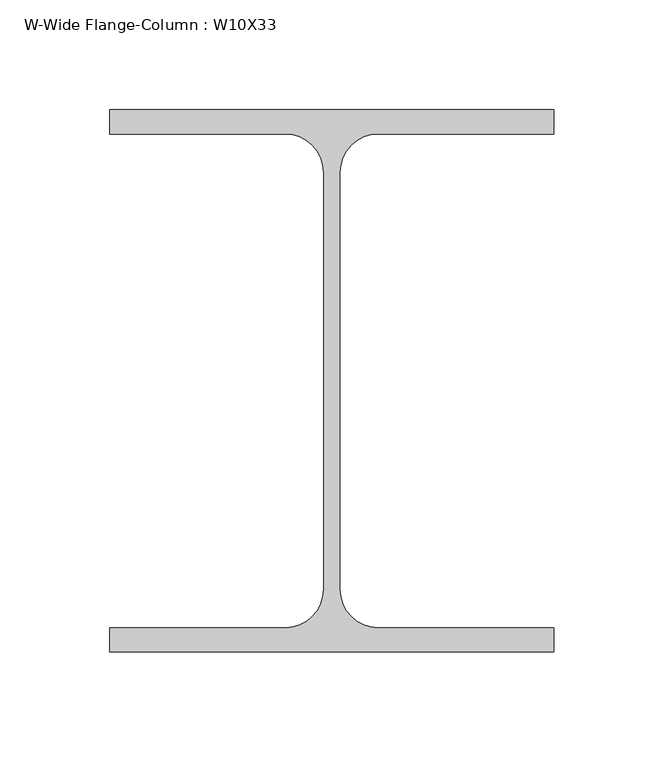
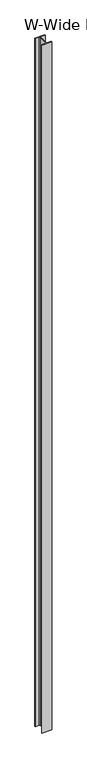
"""IFC4 building model written with IfcOpenShell, lengths in millimetres: column geometry, W-Wide Flange-Column : W10X33."""

import ifcopenshell
import ifcopenshell.guid

model = None  # the IFC model being written
_history = None  # IfcOwnerHistory: only IFC2X3 demands one
_inside = {}  # id of a spatial element -> (the spatial element, [elements in it])
_under = {}  # id of a project, library or spatial element -> (it, [spatial elements below it])
_declared = {}  # id of a project -> (the project, [libraries it declares])
_typed = {}  # id of a type object -> (the type object, [elements of that type])
_made_of = {}  # id of a material, layer set ... -> (it, [elements and type objects made of it])


def new_model(schema):
    """Start an empty IFC model of exactly this schema.

    Asked for "IFC4X3", IfcOpenShell would pick the latest addendum, in which some entities
    have other attributes; the version numbers below select the first issue.
    IFC2X3 requires an IfcOwnerHistory on every rooted entity: one is made here for all.
    """
    global model, _history
    if schema == "IFC4X3":
        model = ifcopenshell.file(schema_version=(4, 3, 0, 0))
    else:
        model = ifcopenshell.file(schema=schema)
    _inside.clear()
    _under.clear()
    _declared.clear()
    _typed.clear()
    _made_of.clear()
    _history = None
    if model.schema == "IFC2X3":
        org = make("IfcOrganization", Name="unknown")
        user = make(
            "IfcPersonAndOrganization",
            ThePerson=make("IfcPerson", FamilyName="unknown"),
            TheOrganization=org,
        )
        app = make(
            "IfcApplication",
            ApplicationDeveloper=org,
            Version="unknown",
            ApplicationFullName="unknown",
            ApplicationIdentifier="unknown",
        )
        _history = make(
            "IfcOwnerHistory",
            OwningUser=user,
            OwningApplication=app,
            ChangeAction="ADDED",
            CreationDate=0,
        )
    return model


def make(cls, **values):
    """One entity of the class cls with the attributes given. An attribute that is None is left unset."""
    return model.create_entity(
        cls, **{name: value for name, value in values.items() if value is not None}
    )


def rooted(cls, **values):
    """An entity with a GlobalId (a new one), such as an element, a storey or a relation."""
    return make(cls, GlobalId=ifcopenshell.guid.new(), OwnerHistory=_history, **values)


def si_unit(unit_type, name, prefix=None):
    """IfcSIUnit, for example si_unit("LENGTHUNIT", "METRE", prefix="MILLI")."""
    return make("IfcSIUnit", UnitType=unit_type, Prefix=prefix, Name=name)


def assignment(units):
    """IfcUnitAssignment: the units of a project."""
    return None if units is None else make("IfcUnitAssignment", Units=units)


def point(xyz):
    """IfcCartesianPoint."""
    return None if xyz is None else make("IfcCartesianPoint", Coordinates=xyz)


def direction(xyz):
    """IfcDirection."""
    return None if xyz is None else make("IfcDirection", DirectionRatios=xyz)


def frame(location, z_axis=None, x_axis=None):
    """IfcAxis2Placement3D, a coordinate frame: its origin and axes. An axis left out is left unset."""
    return make(
        "IfcAxis2Placement3D",
        Location=point(location),
        Axis=direction(z_axis),
        RefDirection=direction(x_axis),
    )


def frame_2d(location, x_axis=None):
    """IfcAxis2Placement2D, a coordinate frame in the plane: its origin and x axis."""
    return make(
        "IfcAxis2Placement2D", Location=point(location), RefDirection=direction(x_axis)
    )


def origin():
    """The frame at (0, 0, 0) with its axes left unset."""
    return frame((0.0, 0.0, 0.0))


def place(relative_to, where):
    """IfcLocalPlacement: puts the frame where relative to a parent placement (None: the world)."""
    return make(
        "IfcLocalPlacement", PlacementRelTo=relative_to, RelativePlacement=where
    )


def context(
    kind, dimensions, precision=None, world=None, true_north=None, identifier=None
):
    """IfcGeometricRepresentationContext, for example the 3D "Model" context."""
    return make(
        "IfcGeometricRepresentationContext",
        ContextIdentifier=identifier,
        ContextType=kind,
        CoordinateSpaceDimension=dimensions,
        Precision=precision,
        WorldCoordinateSystem=world,
        TrueNorth=true_north,
    )


def project(units=None, contexts=None):
    """IfcProject with its units and contexts."""
    return rooted(
        "IfcProject",
        Name="project",
        RepresentationContexts=contexts,
        UnitsInContext=assignment(units),
    )


def spatial(cls, under=None, at=None, **own):
    """A site, building, storey or space (cls), placed at a placement, below another one or the project."""
    s = rooted(cls, ObjectPlacement=at, **own)
    if under is not None:
        _under.setdefault(under.id(), (under, []))[1].append(s)
    return s


def polyline(points):
    """IfcPolyline through the points."""
    return make("IfcPolyline", Points=[point(p) for p in points])


def circle_curve(where, radius):
    """IfcCircle in the frame where."""
    return make("IfcCircle", Position=where, Radius=radius)


def trimmed(basis, trim1, trim2, sense, master):
    """IfcTrimmedCurve: the piece of a basis curve between two trims."""
    return make(
        "IfcTrimmedCurve",
        BasisCurve=basis,
        Trim1=trim1,
        Trim2=trim2,
        SenseAgreement=sense,
        MasterRepresentation=master,
    )


def segment(curve, same_sense, transition):
    """IfcCompositeCurveSegment."""
    return make(
        "IfcCompositeCurveSegment",
        Transition=transition,
        SameSense=same_sense,
        ParentCurve=curve,
    )


def composite_curve(segments, self_intersect=None):
    """IfcCompositeCurve: segments joined end to end."""
    return make("IfcCompositeCurve", Segments=segments, SelfIntersect=self_intersect)


def outline(outer, holes=None, kind="AREA"):
    """IfcArbitraryClosedProfileDef: a profile drawn as a closed curve; with holes, ...WithVoids."""
    if holes is None:
        return make("IfcArbitraryClosedProfileDef", ProfileType=kind, OuterCurve=outer)
    return make(
        "IfcArbitraryProfileDefWithVoids",
        ProfileType=kind,
        OuterCurve=outer,
        InnerCurves=holes,
    )


def extrude(swept, where, along, depth):
    """IfcExtrudedAreaSolid: the profile swept, set in the frame where, extruded along a direction by depth."""
    return make(
        "IfcExtrudedAreaSolid",
        SweptArea=swept,
        Position=where,
        ExtrudedDirection=direction(along),
        Depth=depth,
    )


def shape(context_of_items, identifier, shape_type, items):
    """IfcShapeRepresentation: the items that make up one representation, for example the "Body"."""
    return make(
        "IfcShapeRepresentation",
        ContextOfItems=context_of_items,
        RepresentationIdentifier=identifier,
        RepresentationType=shape_type,
        Items=items,
    )


def source(mapping_origin, context_of_items, identifier, shape_type, items):
    """IfcRepresentationMap: a shape defined once, which mapped items show again and again."""
    return make(
        "IfcRepresentationMap",
        MappingOrigin=mapping_origin,
        MappedRepresentation=shape(context_of_items, identifier, shape_type, items),
    )


def transform(
    local_origin,
    x_axis=None,
    y_axis=None,
    z_axis=None,
    scale=None,
    scale2=None,
    scale3=None,
    uniform=True,
):
    """IfcCartesianTransformationOperator3D, or its non-uniform kind. x_axis, y_axis, z_axis: its Axis1, 2, 3."""
    if uniform:
        return make(
            "IfcCartesianTransformationOperator3D",
            Axis1=direction(x_axis),
            Axis2=direction(y_axis),
            LocalOrigin=point(local_origin),
            Scale=scale,
            Axis3=direction(z_axis),
        )
    return make(
        "IfcCartesianTransformationOperator3DnonUniform",
        Axis1=direction(x_axis),
        Axis2=direction(y_axis),
        LocalOrigin=point(local_origin),
        Scale=scale,
        Axis3=direction(z_axis),
        Scale2=scale2,
        Scale3=scale3,
    )


def mapped(mapping_source, mapping_target):
    """IfcMappedItem: shows the shape of a source again, moved by a transform."""
    return make(
        "IfcMappedItem", MappingSource=mapping_source, MappingTarget=mapping_target
    )


def made_of(thing, what):
    """Note that an element or type object is made of a material, layer set ...; save() writes the relation."""
    if what is not None:
        _made_of.setdefault(what.id(), (what, []))[1].append(thing)
    return thing


def element(
    cls,
    number,
    at=None,
    inside=None,
    cuts=None,
    type_object=None,
    material=None,
    context=None,
    identifier="Body",
    shape_type=None,
    held_by="IfcProductDefinitionShape",
    body=None,
    shapes=None,
    **own,
):
    """One element of the class cls, such as IfcWall. Its Tag is "e" and its number.

    at: its placement. inside: the storey or other place that contains it. cuts: it is an
    opening in that element (IfcRelVoidsElement). A single representation is given by context,
    identifier, shape_type and body (its items); several are given by shapes. held_by: the class
    of the entity that holds the representations. save() writes the other relations.
    """
    e = rooted(cls, Tag="e%d" % number, ObjectPlacement=at, **own)
    if body is not None:
        shapes = [shape(context, identifier, shape_type, body)]
    if shapes is not None:
        e.Representation = make(held_by, Representations=shapes)
    if inside is not None:
        _inside.setdefault(inside.id(), (inside, []))[1].append(e)
    if cuts is not None:
        rooted(
            "IfcRelVoidsElement", RelatingBuildingElement=cuts, RelatedOpeningElement=e
        )
    if type_object is not None:
        _typed.setdefault(type_object.id(), (type_object, []))[1].append(e)
    return made_of(e, material)


def aggregate(whole, parts):
    """IfcRelAggregates: a whole, such as a stair, and the parts it consists of."""
    return rooted("IfcRelAggregates", RelatingObject=whole, RelatedObjects=parts)


def save(model, path):
    """Write the relations noted so far, then the file.

    IfcRelAggregates (storeys below a building ...), IfcRelContainedInSpatialStructure (elements
    in a storey), IfcRelDefinesByType, IfcRelAssociatesMaterial and IfcRelDeclares: one each for
    every whole, place, type object, material and project.
    """
    for whole, parts in _under.values():
        aggregate(whole, parts)
    for where, things in _inside.values():
        rooted(
            "IfcRelContainedInSpatialStructure",
            RelatedElements=things,
            RelatingStructure=where,
        )
    for kind, things in _typed.values():
        rooted("IfcRelDefinesByType", RelatedObjects=things, RelatingType=kind)
    for what, things in _made_of.values():
        rooted("IfcRelAssociatesMaterial", RelatedObjects=things, RelatingMaterial=what)
    for by, libraries in _declared.values():
        rooted("IfcRelDeclares", RelatingContext=by, RelatedDefinitions=libraries)
    model.write(path)


def w_wide_flange_column_w10x33_e941acc0(model_context):
    return source(origin(), model_context, "Body", "SweptSolid", [
        extrude(outline(composite_curve([segment(polyline([(101.092, 123.571), (101.092, 112.522), (21.209, 112.522)]), True, "CONTINUOUS"), segment(trimmed(circle_curve(frame_2d((21.209, 94.996)), 17.526), [point((21.209, 112.522))], [point((3.683, 94.996))], True, "CARTESIAN"), True, "CONTINUOUS"), segment(polyline([(3.683, 94.996), (3.683, -94.996)]), True, "CONTINUOUS"), segment(trimmed(circle_curve(frame_2d((21.209, -94.996)), 17.526), [point((3.683, -94.996))], [point((21.209, -112.522))], True, "CARTESIAN"), True, "CONTINUOUS"), segment(polyline([(21.209, -112.522), (101.092, -112.522), (101.092, -123.571), (-101.092, -123.571), (-101.092, -112.522), (-21.209, -112.522)]), True, "CONTINUOUS"), segment(trimmed(circle_curve(frame_2d((-21.209, -94.996)), 17.526), [point((-21.209, -112.522))], [point((-3.683, -94.996))], True, "CARTESIAN"), True, "CONTINUOUS"), segment(polyline([(-3.683, -94.996), (-3.683, 94.996)]), True, "CONTINUOUS"), segment(trimmed(circle_curve(frame_2d((-21.209, 94.996)), 17.526), [point((-3.683, 94.996))], [point((-21.209, 112.522))], True, "CARTESIAN"), True, "CONTINUOUS"), segment(polyline([(-21.209, 112.522), (-101.092, 112.522), (-101.092, 123.571), (101.092, 123.571)]), True, "CONTINUOUS")], self_intersect=False)), frame((0.0, 0.0, 12566.65), z_axis=(0.0, 0.0, 1.0), x_axis=(1.0, 0.0, 0.0)), (0.0, 0.0, 1.0), 15017.75),
    ])


if __name__ == "__main__":
    model = new_model("IFC4")
    model_context = context("Model", 3, world=origin())
    ifc_project = project(units=[si_unit("LENGTHUNIT", "METRE", prefix="MILLI")], contexts=[model_context])
    site = spatial("IfcSite", under=ifc_project)
    building = spatial("IfcBuilding", under=site)
    placement = place(None, origin())
    w_wide_flange_column_w10x33_shape = w_wide_flange_column_w10x33_e941acc0(model_context)
    element("IfcColumn", 1, ObjectType="W-Wide Flange-Column : W10X33", at=placement, inside=building, context=model_context, shape_type="MappedRepresentation", body=[
        mapped(w_wide_flange_column_w10x33_shape, transform((0.0, 0.0, 0.0), x_axis=(1.0, 0.0, 0.0), y_axis=(0.0, 1.0, 0.0), z_axis=(0.0, 0.0, 1.0))),
    ])
    save(model, "model.ifc")

# Revit data of these elements
# Type "W-Wide Flange-Column : W10X33"
#   Assembly Code = "B10"
#   W = 33
#   bf = 0' - 7.96"
#   d = 0' - 9.73"
#   k = 0' - 1 1/8"
#   kr = 0' - 0.69"
#   tf = 0' - 0.435"
#   tw = 0' - 0.29"
#   A = 0.0674306 SF
#   Structural Material [instance default] = Steel ASTM A992
# Element 1 (IfcColumn, "W-Wide Flange-Column : W10X33")
#   Materials on its faces: "Steel ASTM A992"
# Materials
#   "Steel ASTM A992": class "Metal", colour RGB 199 199 199, transparency 0, Description = "Structural steel 50ksi", Cost = 0
